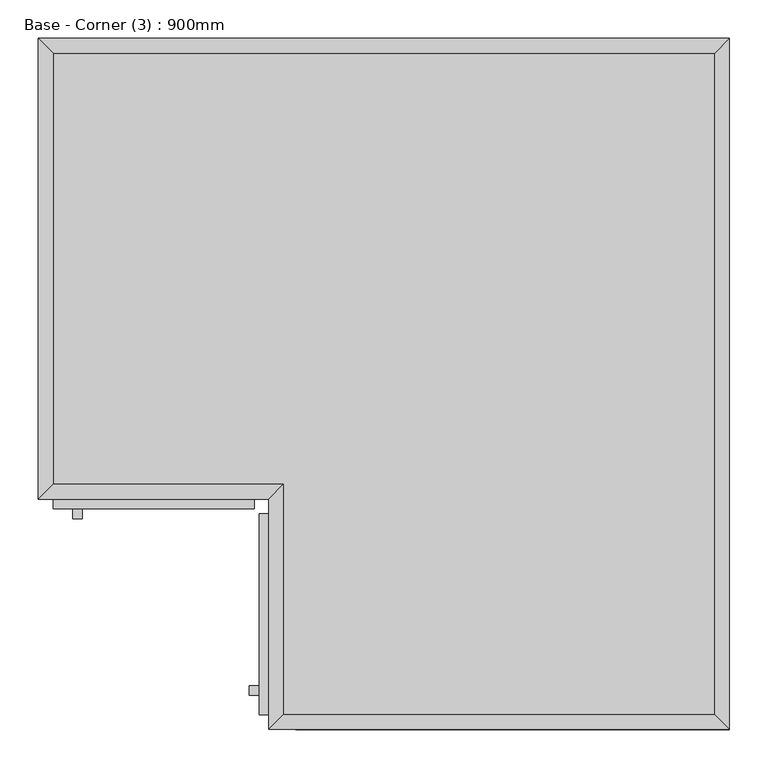
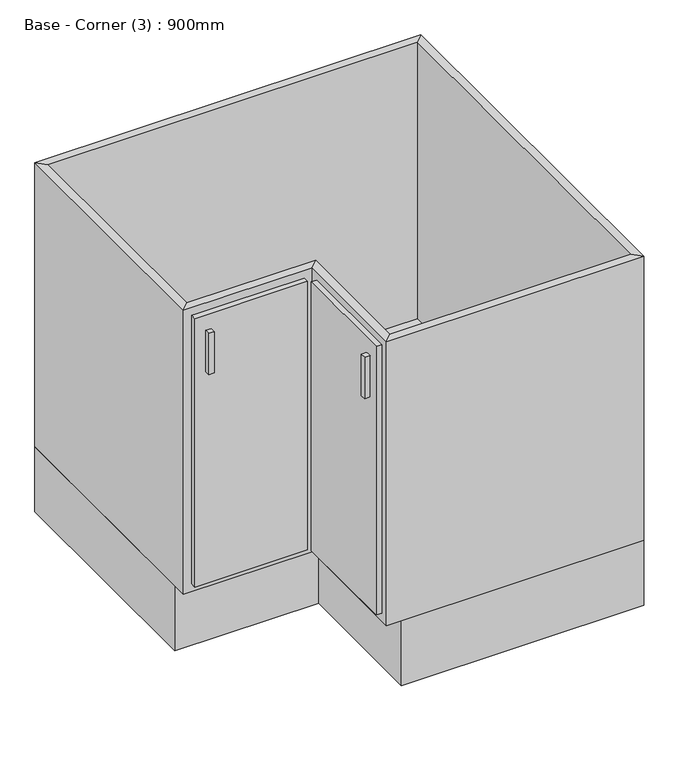
"""IFC4 building model written with IfcOpenShell, lengths in millimetres: furniture geometry, Base - Corner (3) : 900mm."""

from ifc_helpers import new_model, si_unit, frame, origin, origin_with_axes, place, context, project, spatial, polyline, outline, extrude, faceted_brep, source, transform, mapped, element, save


def base_corner_3_900mm_cbc719dc(model_context):
    return source(origin(), model_context, "Body", "SolidModel", [
        extrude(outline(polyline([(-100.3622951, -842.85), (-100.3622951, -855.55), (-113.0622951, -855.55), (-113.0622951, -842.85), (-100.3622951, -842.85)])), frame((0.0, 0.0, 701.25), z_axis=(0.0, 0.0, 1.0), x_axis=(1.0, 0.0, 0.0)), (0.0, 0.0, 1.0), 101.6),
        extrude(outline(polyline([(-87.6622951, -619.05), (-87.6622951, -880.95), (-100.3622951, -880.95), (-100.3622951, -619.05), (-87.6622951, -619.05)])), frame((0.0, 0.0, 179.05), z_axis=(0.0, 0.0, 1.0), x_axis=(1.0, 0.0, 0.0)), (0.0, 0.0, 1.0), 661.9),
        extrude(outline(polyline([(-330.5122951, -625.4), (-343.2122951, -625.4), (-343.2122951, -612.7), (-330.5122951, -612.7), (-330.5122951, -625.4)])), frame((0.0, 0.0, 701.25), z_axis=(0.0, 0.0, 1.0), x_axis=(1.0, 0.0, 0.0)), (0.0, 0.0, 1.0), 101.6),
        extrude(outline(polyline([(-106.7122951, -612.7), (-368.6122951, -612.7), (-368.6122951, -600.0), (-106.7122951, -600.0), (-106.7122951, -612.7)])), frame((0.0, 0.0, 179.05), z_axis=(0.0, 0.0, 1.0), x_axis=(1.0, 0.0, 0.0)), (0.0, 0.0, 1.0), 661.9),
        faceted_brep([(493.2877049, -880.95, 860.0), (493.2877049, -880.95, 160.0), (-68.6122951, -880.95, 160.0), (-68.6122951, -880.95, 860.0), (512.3377049, -900.0, 860.0), (-87.6622951, -900.0, 860.0), (512.3377049, -900.0, 160.0), (-87.6622951, -900.0, 160.0), (-68.6122951, -580.95, 160.0), (-68.6122951, -580.95, 860.0), (-87.6622951, -600.0, 860.0), (-87.6622951, -600.0, 160.0), (-368.6122951, -580.95, 160.0), (-368.6122951, -580.95, 860.0), (-387.6622951, -600.0, 860.0), (-387.6622951, -600.0, 160.0), (-368.6122951, -19.05, 160.0), (-368.6122951, -19.05, 860.0), (-387.6622951, 0.0, 860.0), (-387.6622951, 0.0, 160.0), (493.2877049, -19.05, 160.0), (493.2877049, -19.05, 860.0), (512.3377049, 0.0, 860.0), (512.3377049, 0.0, 160.0)], [[[0, 1, 2, 3]], [[4, 0, 3, 5]], [[6, 4, 5, 7]], [[1, 6, 7, 2]], [[3, 2, 8, 9]], [[5, 3, 9, 10]], [[7, 5, 10, 11]], [[2, 7, 11, 8]], [[9, 8, 12, 13]], [[10, 9, 13, 14]], [[11, 10, 14, 15]], [[8, 11, 15, 12]], [[13, 12, 16, 17]], [[14, 13, 17, 18]], [[15, 14, 18, 19]], [[12, 15, 19, 16]], [[17, 16, 20, 21]], [[18, 17, 21, 22]], [[19, 18, 22, 23]], [[16, 19, 23, 20]], [[21, 20, 1, 0]], [[22, 21, 0, 4]], [[23, 22, 4, 6]], [[20, 23, 6, 1]]]),
        extrude(outline(polyline([(493.2877049, -19.05), (493.2877049, -880.95), (-68.6122951, -880.95), (-68.6122951, -580.95), (-368.6122951, -580.95), (-368.6122951, -19.05), (493.2877049, -19.05)])), frame((0.0, 0.0, 160.0), z_axis=(0.0, 0.0, 1.0), x_axis=(1.0, 0.0, 0.0)), (0.0, 0.0, 1.0), 19.05),
        extrude(outline(polyline([(512.3377049, 0.0), (512.3377049, -900.0), (-52.6622951, -900.0), (-52.6622951, -565.0), (-387.6622951, -565.0), (-387.6622951, 0.0), (512.3377049, 0.0)])), origin_with_axes(), (0.0, 0.0, 1.0), 160.0),
    ])


if __name__ == "__main__":
    model = new_model("IFC4")
    model_context = context("Model", 3, world=origin())
    ifc_project = project(units=[si_unit("LENGTHUNIT", "METRE", prefix="MILLI")], contexts=[model_context])
    site = spatial("IfcSite", under=ifc_project)
    building = spatial("IfcBuilding", under=site)
    placement = place(None, origin())
    base_corner_3_900mm_shape = base_corner_3_900mm_cbc719dc(model_context)
    element("IfcFurniture", 1, ObjectType="Base - Corner (3) : 900mm", at=placement, inside=building, context=model_context, shape_type="MappedRepresentation", body=[
        mapped(base_corner_3_900mm_shape, transform((0.0, 0.0, 0.0), x_axis=(1.0, 0.0, 0.0), y_axis=(0.0, 1.0, 0.0), z_axis=(0.0, 0.0, 1.0))),
    ])
    save(model, "model.ifc")

# Revit data of these elements
# Type "Base - Corner (3) : 900mm"
#   Keynote = "N10"
#   Depth = 600 mm
#   Height = 860 mm
#   Toe Depth = 35 mm
#   Toe Height = 160 mm
#   Width = 900 mm
#   Cabinet Material = Cabinets
#   Door/Drawer Material = Cabinets
#   Handle Material = Cabinets - Handles
#   Assembly Code = ""
# Element 1 (IfcFurniture, "Base - Corner (3) : 900mm")
#   Materials on its faces: "Cabinets", "Cabinets - Handles"
# Materials
#   "Cabinets": class "Miscellaneous", colour RGB 249 249 249, transparency 0
#   "Cabinets - Handles": class "Metal", colour RGB 57 57 57, transparency 0
